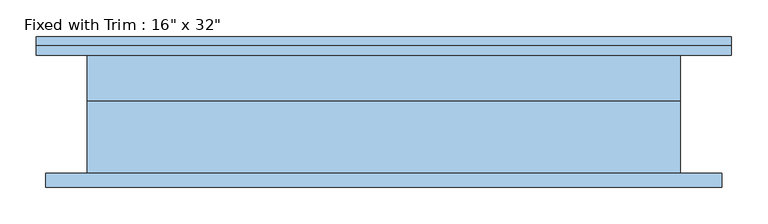
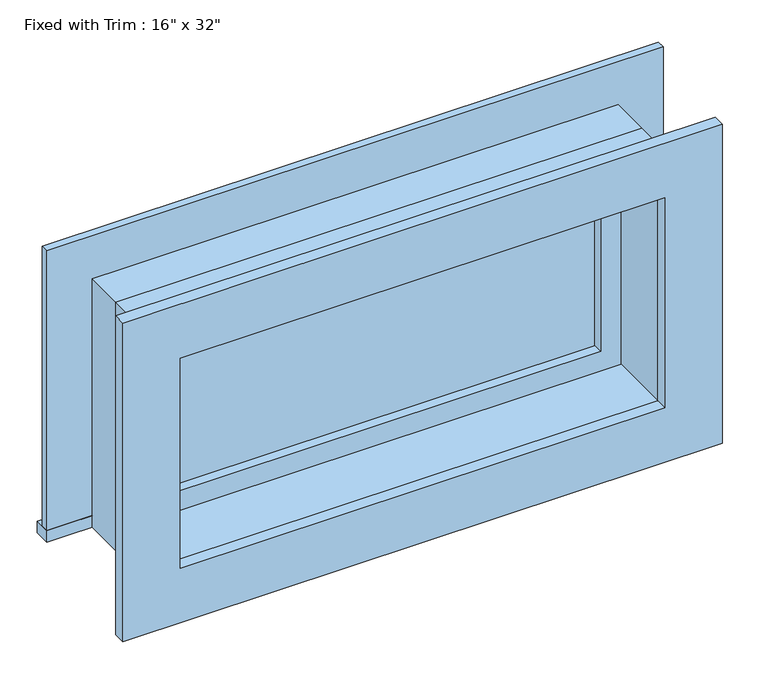
"""IFC4 building model written with IfcOpenShell, lengths in millimetres: window geometry."""

from ifc_helpers import new_model, si_unit, frame, origin, place, context, project, spatial, polyline, outline, extrude, source, transform, mapped, element, save


def window_31fe39a7(model_context):
    return source(origin(), model_context, "Body", "SweptSolid", [
        extrude(outline(polyline([(-514.35, 106.3625), (438.15, 106.3625), (438.15, 80.9625), (-514.35, 80.9625), (-514.35, 106.3625)])), frame((0.0, 0.0, 914.4), z_axis=(0.0, 0.0, 1.0), x_axis=(1.0, 0.0, 0.0)), (0.0, 0.0, 1.0), 19.05),
        extrude(outline(polyline([(1301.75, -425.45), (1301.75, 349.25), (933.45, 349.25), (933.45, 438.15), (1390.65, 438.15), (1390.65, -514.35), (933.45, -514.35), (933.45, -425.45), (1301.75, -425.45)])), frame((0.0, 80.9625, 0.0), z_axis=(0.0, 1.0, 0.0), x_axis=(0.0, 0.0, 1.0)), (0.0, 0.0, 1.0), 12.7),
        extrude(outline(polyline([(1377.95, 425.45), (1377.95, -501.65), (857.25, -501.65), (857.25, 425.45), (1377.95, 425.45)]), holes=[polyline([(1289.05, 336.55), (946.15, 336.55), (946.15, -412.75), (1289.05, -412.75), (1289.05, 336.55)])]), frame((0.0, -100.0125, 0.0), z_axis=(0.0, 1.0, 0.0), x_axis=(0.0, 0.0, 1.0)), (0.0, 0.0, 1.0), 19.05),
        extrude(outline(polyline([(304.8, 33.3375), (-381.0, 33.3375), (-381.0, 46.0375), (304.8, 46.0375), (304.8, 33.3375)])), frame((0.0, 0.0, 977.9), z_axis=(0.0, 0.0, 1.0), x_axis=(1.0, 0.0, 0.0)), (0.0, 0.0, 1.0), 279.4),
        extrude(outline(polyline([(1301.75, -425.45), (933.45, -425.45), (933.45, 349.25), (1301.75, 349.25), (1301.75, -425.45)]), holes=[polyline([(1257.3, -381.0), (1257.3, 304.8), (977.9, 304.8), (977.9, -381.0), (1257.3, -381.0)])]), frame((0.0, 17.4625, 0.0), z_axis=(0.0, 1.0, 0.0), x_axis=(0.0, 0.0, 1.0)), (0.0, 0.0, 1.0), 44.45),
        extrude(outline(polyline([(1320.8, -444.5), (914.4, -444.5), (914.4, 368.3), (1320.8, 368.3), (1320.8, -444.5)]), holes=[polyline([(1289.05, -412.75), (1289.05, 336.55), (946.15, 336.55), (946.15, -412.75), (1289.05, -412.75)])]), frame((0.0, -80.9625, 0.0), z_axis=(0.0, 1.0, 0.0), x_axis=(0.0, 0.0, 1.0)), (0.0, 0.0, 1.0), 98.425),
        extrude(outline(polyline([(1320.8, 368.3), (1320.8, -444.5), (914.4, -444.5), (914.4, 368.3), (1320.8, 368.3)]), holes=[polyline([(1301.75, 349.25), (933.45, 349.25), (933.45, -425.45), (1301.75, -425.45), (1301.75, 349.25)])]), frame((0.0, 17.4625, 0.0), z_axis=(0.0, 1.0, 0.0), x_axis=(0.0, 0.0, 1.0)), (0.0, 0.0, 1.0), 63.5),
    ])


if __name__ == "__main__":
    model = new_model("IFC4")
    model_context = context("Model", 3, world=origin())
    ifc_project = project(units=[si_unit("LENGTHUNIT", "METRE", prefix="MILLI")], contexts=[model_context])
    site = spatial("IfcSite", under=ifc_project)
    building = spatial("IfcBuilding", under=site)
    placement = place(None, origin())
    window_shape = window_31fe39a7(model_context)
    element("IfcWindow", 1, ObjectType="Fixed with Trim : 16\" x 32\"", at=placement, inside=building, context=model_context, shape_type="MappedRepresentation", body=[
        mapped(window_shape, transform((0.0, 0.0, 0.0), x_axis=(1.0, 0.0, 0.0), y_axis=(0.0, 1.0, 0.0), z_axis=(0.0, 0.0, 1.0))),
    ])
    save(model, "model.ifc")

# Revit data of these elements
# Type "Fixed with Trim : 16\" x 32\""
#   Type Mark = "64"
#   COBie.Type.CreatedBy = "doug.wood@us.ibm.com"
#   COBie.Type.CreatedOn = "2016-04-14T02:07:26"
#   COBie.Type.Name = "Windows_Fixed with Trim_16\" x 32\"_64"
#   COBie.Type.Category = "23-30 20 17 11 : Fixed Windows"
#   COBie.Type.Description = "Fixed with Trim_16\" x 32\""
#   COBie.Type.Manufacturer = ""
#   COBie.Type.ModelNumber = ""
#   Construction Type Id = "GSP4R"
#   Assembly Code = "B2020100"
#   Analytic Construction = "1/8 in Pilkington single glazing"
#   COBie.Type.ReplacementCost = 0
#   Visual Light Transmittance = 0.9
#   Solar Heat Gain Coefficient = 0.78
#   Heat Transfer Coefficient (U) = 3.6886 W/(m²·K)
#   Height = 1' - 4"
#   Default Sill Height = 3' - 0"
#   Trim Projection - Ext. = 0' - 0 1/2"
#   Trim Projection - Int. = 0' - 0 3/4"
#   Trim Width - Exterior = 0' - 3 1/2"
#   Trim Width - Interior = 0' - 3 1/2"
#   Width = 2' - 8"
#   Window Inset = 0' - 0 3/4"
#   COBie.Type = no
#   Glass Pane Material = Glass
#   Sash Material = Sash - White
#   Trim Exterior Material = Trim - White
#   Trim Interior Material = Trim - White
#   Wall Closure = (empty or 0)
# Element 1 (IfcWindow, "Fixed with Trim : 16\" x 32\"")
#   Materials on its faces: "Sash - White", "Trim - White", "Glass"
# Materials
#   "Glass": class "Glass", colour RGB 0 128 192, transparency 0.75, Description = "Soda Lime Glass", Cost = 0
#   "Sash - White": class "Wood", colour RGB 255 255 255, transparency 0, Cost = 0
#   "Trim - White": class "Wood", colour RGB 255 255 255, transparency 0, Cost = 0
